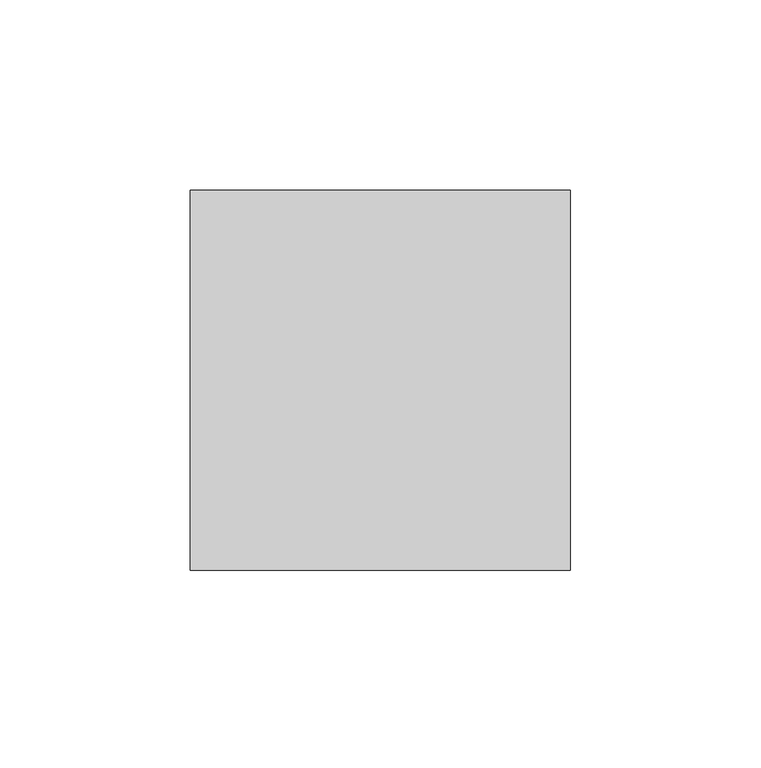
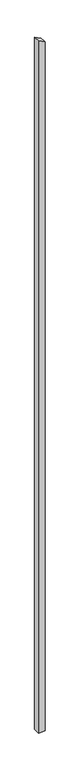
"""IFC4 building model written with IfcOpenShell, lengths in millimetres: column geometry, Holzstütze 159656 : Holzstütze 159656."""

from ifc_helpers import new_model, si_unit, frame, origin, place, context, project, spatial, polyline, outline, extrude, source, transform, mapped, element, save


def column_c1a18ea8(model_context):
    return source(origin(), model_context, "Body", "SweptSolid", [
        extrude(outline(polyline([(-500.0, 165867.7593015), (-500.0, 165967.7593015), (10590.0588201, 165967.7593015), (10641.011365, 165867.7593015), (-500.0, 165867.7593015)])), frame((0.0, 26981.9343946, 0.0), z_axis=(0.0, 1.0, 0.0), x_axis=(0.0, 0.0, 1.0)), (0.0, 0.0, 1.0), 100.0),
    ])


if __name__ == "__main__":
    model = new_model("IFC4")
    model_context = context("Model", 3, world=origin())
    ifc_project = project(units=[si_unit("LENGTHUNIT", "METRE", prefix="MILLI")], contexts=[model_context])
    site = spatial("IfcSite", under=ifc_project)
    building = spatial("IfcBuilding", under=site)
    placement = place(None, origin())
    column_shape = column_c1a18ea8(model_context)
    element("IfcColumn", 1, ObjectType="Holzstütze 159656 : Holzstütze 159656", at=placement, inside=building, context=model_context, shape_type="MappedRepresentation", body=[
        mapped(column_shape, transform((0.0, 0.0, 0.0), x_axis=(1.0, 0.0, 0.0), y_axis=(0.0, 1.0, 0.0), z_axis=(0.0, 0.0, 1.0))),
    ])
    save(model, "model.ifc")

# Revit data of these elements
# Type "Holzstütze 159656 : Holzstütze 159656"
#   Abrechnungsart = "m"
#   Allright_Bauteil_ID = "0152St 0000143519"
#   Bezeichnung = "Holzstütze"
#   Codetext = "ST-HOLZ\\"
#   Gewerk = "Zimmer- und Holzbauarbeiten"
#   Material = "Holz"
#   Objektname = "Stütze"
#   NameOverride = "Holzstütze"
#   Reference = "Holzstütze"
#   Status = "NEW"
#   ThermalTransmittance = 0.0000 BTU/(h·ft²·°F)
#   Roll = 0.00°
#   Slope = 0.00°
#   2D Interaktion = yes
#   IsExternal = yes
#   LoadBearing = yes
# Element 1 (IfcColumn, "Holzstütze 159656 : Holzstütze 159656")
#   Materials on its faces: "holzschalung"
# Materials
#   "holzschalung": class "Unassigned", colour RGB 128 128 128, transparency 0
